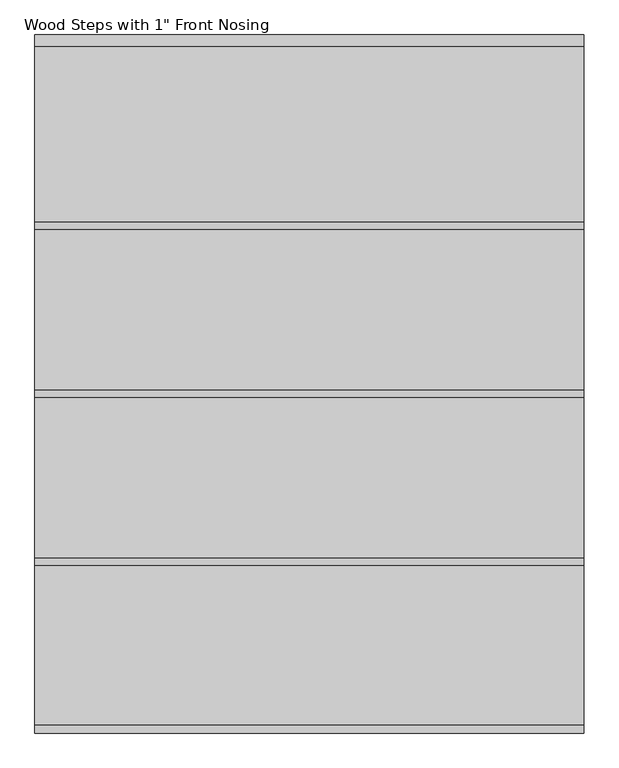
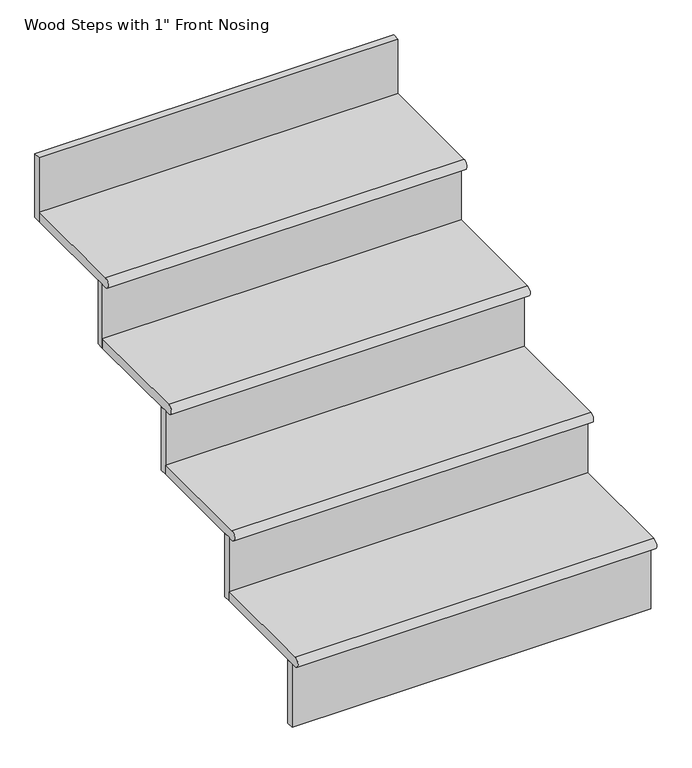
"""IFC4 building model written with IfcOpenShell, lengths in millimetres: stair flight geometry."""

import ifcopenshell
import ifcopenshell.guid

model = None  # the IFC model being written
_history = None  # IfcOwnerHistory: only IFC2X3 demands one
_inside = {}  # id of a spatial element -> (the spatial element, [elements in it])
_under = {}  # id of a project, library or spatial element -> (it, [spatial elements below it])
_declared = {}  # id of a project -> (the project, [libraries it declares])
_typed = {}  # id of a type object -> (the type object, [elements of that type])
_made_of = {}  # id of a material, layer set ... -> (it, [elements and type objects made of it])


def new_model(schema):
    """Start an empty IFC model of exactly this schema.

    Asked for "IFC4X3", IfcOpenShell would pick the latest addendum, in which some entities
    have other attributes; the version numbers below select the first issue.
    IFC2X3 requires an IfcOwnerHistory on every rooted entity: one is made here for all.
    """
    global model, _history
    if schema == "IFC4X3":
        model = ifcopenshell.file(schema_version=(4, 3, 0, 0))
    else:
        model = ifcopenshell.file(schema=schema)
    _inside.clear()
    _under.clear()
    _declared.clear()
    _typed.clear()
    _made_of.clear()
    _history = None
    if model.schema == "IFC2X3":
        org = make("IfcOrganization", Name="unknown")
        user = make(
            "IfcPersonAndOrganization",
            ThePerson=make("IfcPerson", FamilyName="unknown"),
            TheOrganization=org,
        )
        app = make(
            "IfcApplication",
            ApplicationDeveloper=org,
            Version="unknown",
            ApplicationFullName="unknown",
            ApplicationIdentifier="unknown",
        )
        _history = make(
            "IfcOwnerHistory",
            OwningUser=user,
            OwningApplication=app,
            ChangeAction="ADDED",
            CreationDate=0,
        )
    return model


def make(cls, **values):
    """One entity of the class cls with the attributes given. An attribute that is None is left unset."""
    return model.create_entity(
        cls, **{name: value for name, value in values.items() if value is not None}
    )


def rooted(cls, **values):
    """An entity with a GlobalId (a new one), such as an element, a storey or a relation."""
    return make(cls, GlobalId=ifcopenshell.guid.new(), OwnerHistory=_history, **values)


def si_unit(unit_type, name, prefix=None):
    """IfcSIUnit, for example si_unit("LENGTHUNIT", "METRE", prefix="MILLI")."""
    return make("IfcSIUnit", UnitType=unit_type, Prefix=prefix, Name=name)


def assignment(units):
    """IfcUnitAssignment: the units of a project."""
    return None if units is None else make("IfcUnitAssignment", Units=units)


def point(xyz):
    """IfcCartesianPoint."""
    return None if xyz is None else make("IfcCartesianPoint", Coordinates=xyz)


def direction(xyz):
    """IfcDirection."""
    return None if xyz is None else make("IfcDirection", DirectionRatios=xyz)


def frame(location, z_axis=None, x_axis=None):
    """IfcAxis2Placement3D, a coordinate frame: its origin and axes. An axis left out is left unset."""
    return make(
        "IfcAxis2Placement3D",
        Location=point(location),
        Axis=direction(z_axis),
        RefDirection=direction(x_axis),
    )


def frame_2d(location, x_axis=None):
    """IfcAxis2Placement2D, a coordinate frame in the plane: its origin and x axis."""
    return make(
        "IfcAxis2Placement2D", Location=point(location), RefDirection=direction(x_axis)
    )


def origin():
    """The frame at (0, 0, 0) with its axes left unset."""
    return frame((0.0, 0.0, 0.0))


def place(relative_to, where):
    """IfcLocalPlacement: puts the frame where relative to a parent placement (None: the world)."""
    return make(
        "IfcLocalPlacement", PlacementRelTo=relative_to, RelativePlacement=where
    )


def context(
    kind, dimensions, precision=None, world=None, true_north=None, identifier=None
):
    """IfcGeometricRepresentationContext, for example the 3D "Model" context."""
    return make(
        "IfcGeometricRepresentationContext",
        ContextIdentifier=identifier,
        ContextType=kind,
        CoordinateSpaceDimension=dimensions,
        Precision=precision,
        WorldCoordinateSystem=world,
        TrueNorth=true_north,
    )


def project(units=None, contexts=None):
    """IfcProject with its units and contexts."""
    return rooted(
        "IfcProject",
        Name="project",
        RepresentationContexts=contexts,
        UnitsInContext=assignment(units),
    )


def spatial(cls, under=None, at=None, **own):
    """A site, building, storey or space (cls), placed at a placement, below another one or the project."""
    s = rooted(cls, ObjectPlacement=at, **own)
    if under is not None:
        _under.setdefault(under.id(), (under, []))[1].append(s)
    return s


def polyline(points):
    """IfcPolyline through the points."""
    return make("IfcPolyline", Points=[point(p) for p in points])


def circle_curve(where, radius):
    """IfcCircle in the frame where."""
    return make("IfcCircle", Position=where, Radius=radius)


def trimmed(basis, trim1, trim2, sense, master):
    """IfcTrimmedCurve: the piece of a basis curve between two trims."""
    return make(
        "IfcTrimmedCurve",
        BasisCurve=basis,
        Trim1=trim1,
        Trim2=trim2,
        SenseAgreement=sense,
        MasterRepresentation=master,
    )


def segment(curve, same_sense, transition):
    """IfcCompositeCurveSegment."""
    return make(
        "IfcCompositeCurveSegment",
        Transition=transition,
        SameSense=same_sense,
        ParentCurve=curve,
    )


def composite_curve(segments, self_intersect=None):
    """IfcCompositeCurve: segments joined end to end."""
    return make("IfcCompositeCurve", Segments=segments, SelfIntersect=self_intersect)


def outline(outer, holes=None, kind="AREA"):
    """IfcArbitraryClosedProfileDef: a profile drawn as a closed curve; with holes, ...WithVoids."""
    if holes is None:
        return make("IfcArbitraryClosedProfileDef", ProfileType=kind, OuterCurve=outer)
    return make(
        "IfcArbitraryProfileDefWithVoids",
        ProfileType=kind,
        OuterCurve=outer,
        InnerCurves=holes,
    )


def extrude(swept, where, along, depth):
    """IfcExtrudedAreaSolid: the profile swept, set in the frame where, extruded along a direction by depth."""
    return make(
        "IfcExtrudedAreaSolid",
        SweptArea=swept,
        Position=where,
        ExtrudedDirection=direction(along),
        Depth=depth,
    )


def shape(context_of_items, identifier, shape_type, items):
    """IfcShapeRepresentation: the items that make up one representation, for example the "Body"."""
    return make(
        "IfcShapeRepresentation",
        ContextOfItems=context_of_items,
        RepresentationIdentifier=identifier,
        RepresentationType=shape_type,
        Items=items,
    )


def source(mapping_origin, context_of_items, identifier, shape_type, items):
    """IfcRepresentationMap: a shape defined once, which mapped items show again and again."""
    return make(
        "IfcRepresentationMap",
        MappingOrigin=mapping_origin,
        MappedRepresentation=shape(context_of_items, identifier, shape_type, items),
    )


def transform(
    local_origin,
    x_axis=None,
    y_axis=None,
    z_axis=None,
    scale=None,
    scale2=None,
    scale3=None,
    uniform=True,
):
    """IfcCartesianTransformationOperator3D, or its non-uniform kind. x_axis, y_axis, z_axis: its Axis1, 2, 3."""
    if uniform:
        return make(
            "IfcCartesianTransformationOperator3D",
            Axis1=direction(x_axis),
            Axis2=direction(y_axis),
            LocalOrigin=point(local_origin),
            Scale=scale,
            Axis3=direction(z_axis),
        )
    return make(
        "IfcCartesianTransformationOperator3DnonUniform",
        Axis1=direction(x_axis),
        Axis2=direction(y_axis),
        LocalOrigin=point(local_origin),
        Scale=scale,
        Axis3=direction(z_axis),
        Scale2=scale2,
        Scale3=scale3,
    )


def mapped(mapping_source, mapping_target):
    """IfcMappedItem: shows the shape of a source again, moved by a transform."""
    return make(
        "IfcMappedItem", MappingSource=mapping_source, MappingTarget=mapping_target
    )


def made_of(thing, what):
    """Note that an element or type object is made of a material, layer set ...; save() writes the relation."""
    if what is not None:
        _made_of.setdefault(what.id(), (what, []))[1].append(thing)
    return thing


def element(
    cls,
    number,
    at=None,
    inside=None,
    cuts=None,
    type_object=None,
    material=None,
    context=None,
    identifier="Body",
    shape_type=None,
    held_by="IfcProductDefinitionShape",
    body=None,
    shapes=None,
    **own,
):
    """One element of the class cls, such as IfcWall. Its Tag is "e" and its number.

    at: its placement. inside: the storey or other place that contains it. cuts: it is an
    opening in that element (IfcRelVoidsElement). A single representation is given by context,
    identifier, shape_type and body (its items); several are given by shapes. held_by: the class
    of the entity that holds the representations. save() writes the other relations.
    """
    e = rooted(cls, Tag="e%d" % number, ObjectPlacement=at, **own)
    if body is not None:
        shapes = [shape(context, identifier, shape_type, body)]
    if shapes is not None:
        e.Representation = make(held_by, Representations=shapes)
    if inside is not None:
        _inside.setdefault(inside.id(), (inside, []))[1].append(e)
    if cuts is not None:
        rooted(
            "IfcRelVoidsElement", RelatingBuildingElement=cuts, RelatedOpeningElement=e
        )
    if type_object is not None:
        _typed.setdefault(type_object.id(), (type_object, []))[1].append(e)
    return made_of(e, material)


def aggregate(whole, parts):
    """IfcRelAggregates: a whole, such as a stair, and the parts it consists of."""
    return rooted("IfcRelAggregates", RelatingObject=whole, RelatedObjects=parts)


def save(model, path):
    """Write the relations noted so far, then the file.

    IfcRelAggregates (storeys below a building ...), IfcRelContainedInSpatialStructure (elements
    in a storey), IfcRelDefinesByType, IfcRelAssociatesMaterial and IfcRelDeclares: one each for
    every whole, place, type object, material and project.
    """
    for whole, parts in _under.values():
        aggregate(whole, parts)
    for where, things in _inside.values():
        rooted(
            "IfcRelContainedInSpatialStructure",
            RelatedElements=things,
            RelatingStructure=where,
        )
    for kind, things in _typed.values():
        rooted("IfcRelDefinesByType", RelatedObjects=things, RelatingType=kind)
    for what, things in _made_of.values():
        rooted("IfcRelAssociatesMaterial", RelatedObjects=things, RelatingMaterial=what)
    for by, libraries in _declared.values():
        rooted("IfcRelDeclares", RelatingContext=by, RelatedDefinitions=libraries)
    model.write(path)


def stair_flight_4bcf9645(model_context):
    return source(origin(), model_context, "Body", "SweptSolid", [
        extrude(outline(composite_curve([segment(polyline([(-12436.2557429, 4629.15), (-12144.1557429, 4629.15), (-12144.1557429, 4603.75), (-12436.2557429, 4603.75)]), True, "CONTINUOUS"), segment(trimmed(circle_curve(frame_2d((-12436.2557429, 4616.45)), 12.7), [point((-12436.2557429, 4603.75))], [point((-12436.2557429, 4629.15))], False, "CARTESIAN"), True, "CONTINUOUS")], self_intersect=False)), frame((6489.8789345, 0.0, 0.0), z_axis=(1.0, 0.0, 0.0), x_axis=(0.0, 1.0, 0.0)), (0.0, 0.0, 1.0), 914.4),
        extrude(outline(polyline([(7404.2789345, -12404.5057429), (7404.2789345, -12423.5557429), (6489.8789345, -12423.5557429), (6489.8789345, -12404.5057429), (7404.2789345, -12404.5057429)])), frame((0.0, 0.0, 4432.3), z_axis=(0.0, 0.0, 1.0), x_axis=(1.0, 0.0, 0.0)), (0.0, 0.0, 1.0), 171.45),
        extrude(outline(polyline([(7404.2789345, -12125.1057429), (7404.2789345, -12144.1557429), (6489.8789345, -12144.1557429), (6489.8789345, -12125.1057429), (7404.2789345, -12125.1057429)])), frame((0.0, 0.0, 4603.75), z_axis=(0.0, 0.0, 1.0), x_axis=(1.0, 0.0, 0.0)), (0.0, 0.0, 1.0), 171.45),
        extrude(outline(composite_curve([segment(polyline([(-12156.8557429, 4800.6), (-11864.7557429, 4800.6), (-11864.7557429, 4775.2), (-12156.8557429, 4775.2)]), True, "CONTINUOUS"), segment(trimmed(circle_curve(frame_2d((-12156.8557429, 4787.9)), 12.7), [point((-12156.8557429, 4775.2))], [point((-12156.8557429, 4800.6))], False, "CARTESIAN"), True, "CONTINUOUS")], self_intersect=False)), frame((6489.8789345, 0.0, 0.0), z_axis=(1.0, 0.0, 0.0), x_axis=(0.0, 1.0, 0.0)), (0.0, 0.0, 1.0), 914.4),
        extrude(outline(polyline([(7404.2789345, -11845.7057429), (7404.2789345, -11864.7557429), (6489.8789345, -11864.7557429), (6489.8789345, -11845.7057429), (7404.2789345, -11845.7057429)])), frame((0.0, 0.0, 4775.2), z_axis=(0.0, 0.0, 1.0), x_axis=(1.0, 0.0, 0.0)), (0.0, 0.0, 1.0), 171.45),
        extrude(outline(composite_curve([segment(polyline([(-11877.4557429, 4972.05), (-11585.3557429, 4972.05), (-11585.3557429, 4946.65), (-11877.4557429, 4946.65)]), True, "CONTINUOUS"), segment(trimmed(circle_curve(frame_2d((-11877.4557429, 4959.35)), 12.7), [point((-11877.4557429, 4946.65))], [point((-11877.4557429, 4972.05))], False, "CARTESIAN"), True, "CONTINUOUS")], self_intersect=False)), frame((6489.8789345, 0.0, 0.0), z_axis=(1.0, 0.0, 0.0), x_axis=(0.0, 1.0, 0.0)), (0.0, 0.0, 1.0), 914.4),
        extrude(outline(polyline([(7404.2789345, -11566.3057429), (7404.2789345, -11585.3557429), (6489.8789345, -11585.3557429), (6489.8789345, -11566.3057429), (7404.2789345, -11566.3057429)])), frame((0.0, 0.0, 4946.65), z_axis=(0.0, 0.0, 1.0), x_axis=(1.0, 0.0, 0.0)), (0.0, 0.0, 1.0), 171.45),
        extrude(outline(polyline([(7404.2789345, -11286.9057429), (7404.2789345, -11305.9557429), (6489.8789345, -11305.9557429), (6489.8789345, -11286.9057429), (7404.2789345, -11286.9057429)])), frame((0.0, 0.0, 5118.1), z_axis=(0.0, 0.0, 1.0), x_axis=(1.0, 0.0, 0.0)), (0.0, 0.0, 1.0), 171.45),
        extrude(outline(composite_curve([segment(polyline([(-11598.0557429, 5143.5), (-11305.9557429, 5143.5), (-11305.9557429, 5118.1), (-11598.0557429, 5118.1)]), True, "CONTINUOUS"), segment(trimmed(circle_curve(frame_2d((-11598.0557429, 5130.8)), 12.7), [point((-11598.0557429, 5118.1))], [point((-11598.0557429, 5143.5))], False, "CARTESIAN"), True, "CONTINUOUS")], self_intersect=False)), frame((6489.8789345, 0.0, 0.0), z_axis=(1.0, 0.0, 0.0), x_axis=(0.0, 1.0, 0.0)), (0.0, 0.0, 1.0), 914.4),
    ])


if __name__ == "__main__":
    model = new_model("IFC4")
    model_context = context("Model", 3, world=origin())
    ifc_project = project(units=[si_unit("LENGTHUNIT", "METRE", prefix="MILLI")], contexts=[model_context])
    site = spatial("IfcSite", under=ifc_project)
    building = spatial("IfcBuilding", under=site)
    placement = place(None, origin())
    stair_flight_shape = stair_flight_4bcf9645(model_context)
    element("IfcStairFlight", 1, ObjectType="Wood Steps with 1\" Front Nosing", at=placement, inside=building, context=model_context, shape_type="MappedRepresentation", body=[
        mapped(stair_flight_shape, transform((0.0, 0.0, 0.0), x_axis=(1.0, 0.0, 0.0), y_axis=(0.0, 1.0, 0.0), z_axis=(0.0, 0.0, 1.0))),
    ])
    save(model, "model.ifc")

# Revit data of these elements
# Element 1 (IfcStairFlight, "Wood Steps with 1\" Front Nosing")
#   Materials on its faces: "Paints and Coatings", "Cherry"
# Materials
#   "Paints and Coatings": class "Paint", colour RGB 244 244 244, transparency 0, Description = "Interior finish", Cost = 0
#   "Cherry": class "Wood", colour RGB 233 182 144, transparency 0, Description = "Prunus Serotina", Cost = 0
